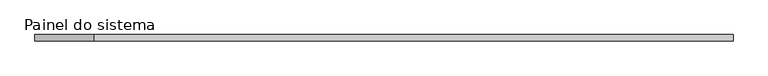
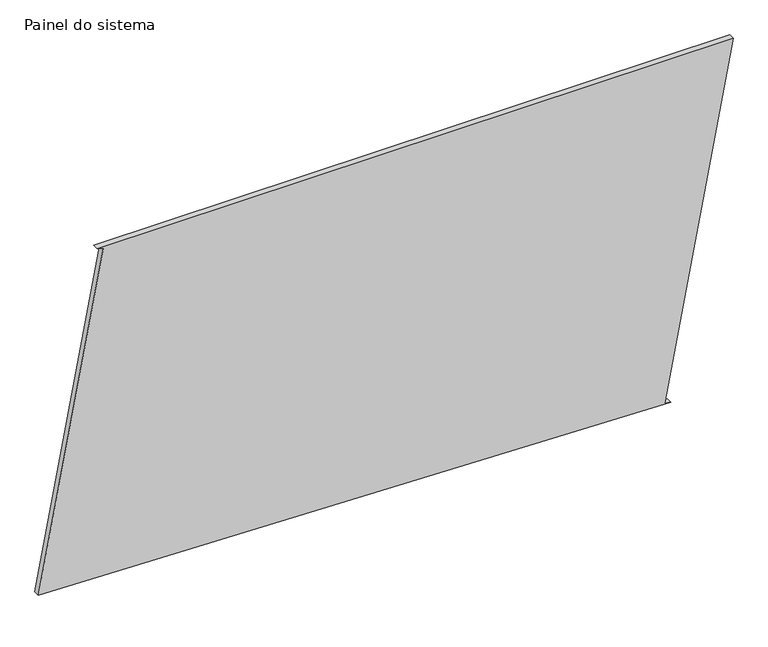
"""IFC4 building model written with IfcOpenShell, lengths in millimetres: plate geometry, Painel do sistema : Envidraçado."""

from ifc_helpers import new_model, si_unit, frame, origin, place, context, project, spatial, polyline, outline, extrude, source, transform, mapped, element, save


def painel_do_sistema_9743723e(model_context):
    return source(origin(), model_context, "Body", "SweptSolid", [
        extrude(outline(polyline([(0.0, 1162.6842147), (4.6288169, 1138.1164706), (1480.2516345, 1416.139059), (1480.2516345, -1176.3139959), (1475.6228176, -1151.7462517), (72.3409423, -1416.139059), (0.0, 1162.6842147)])), frame((0.0, 24.5, 0.0), z_axis=(0.0, 1.0, 0.0), x_axis=(0.0, 0.0, 1.0)), (0.0, 0.0, 1.0), 25.0),
    ])


if __name__ == "__main__":
    model = new_model("IFC4")
    model_context = context("Model", 3, world=origin())
    ifc_project = project(units=[si_unit("LENGTHUNIT", "METRE", prefix="MILLI")], contexts=[model_context])
    site = spatial("IfcSite", under=ifc_project)
    building = spatial("IfcBuilding", under=site)
    placement = place(None, origin())
    painel_do_sistema_shape = painel_do_sistema_9743723e(model_context)
    element("IfcPlate", 1, ObjectType="Painel do sistema : Envidraçado", at=placement, inside=building, context=model_context, shape_type="MappedRepresentation", body=[
        mapped(painel_do_sistema_shape, transform((0.0, 0.0, 0.0), x_axis=(1.0, 0.0, 0.0), y_axis=(0.0, 1.0, 0.0), z_axis=(0.0, 0.0, 1.0))),
    ])
    save(model, "model.ifc")

# Revit data of these elements
# Type "Painel do sistema : Envidraçado"
#   Construction Type Id = "GSP4R"
#   Analytic Construction = "Vidraça única Pilkington 1/8 pol"
#   Visual Light Transmittance = 0.9
#   Solar Heat Gain Coefficient = 0.86
#   Heat Transfer Coefficient (U) = 6.7069 W/(m²·K)
# Element 1 (IfcPlate, "Painel do sistema : Envidraçado")
#   Materials on its faces: "Vidro"
# Materials
#   "Vidro": class "Vidro", colour RGB 0 128 192, transparency 0.9, Description = "Vidro de sílica", Cost = 0
